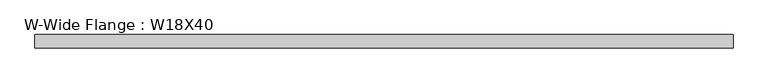
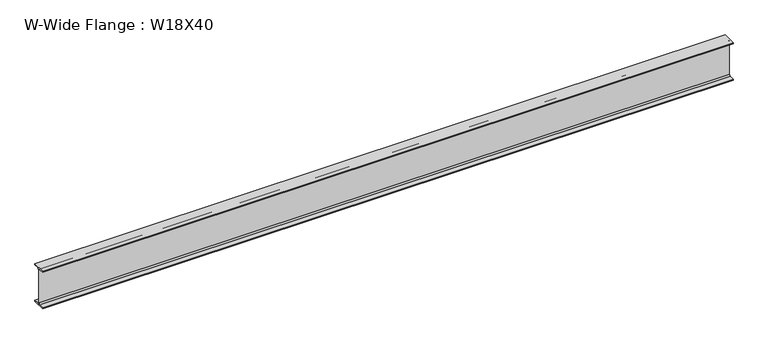
"""IFC4 building model written with IfcOpenShell, lengths in millimetres: beam geometry, W-Wide Flange : W18X40."""

from ifc_helpers import new_model, si_unit, point, frame, frame_2d, origin, place, context, project, spatial, polyline, circle_curve, trimmed, segment, composite_curve, outline, extrude, source, transform, mapped, element, save


def w_wide_flange_w18x40_d8d7ebc0(model_context):
    return source(origin(), model_context, "Body", "SweptSolid", [
        extrude(outline(composite_curve([segment(polyline([(76.454, -213.995), (76.454, -227.33), (-76.454, -227.33), (-76.454, -213.995), (-20.828, -213.995)]), True, "CONTINUOUS"), segment(trimmed(circle_curve(frame_2d((-20.828, -197.1675)), 16.8275), [point((-20.828, -213.995))], [point((-4.0005, -197.1675))], True, "CARTESIAN"), True, "CONTINUOUS"), segment(polyline([(-4.0005, -197.1675), (-4.0005, 197.1675)]), True, "CONTINUOUS"), segment(trimmed(circle_curve(frame_2d((-20.828, 197.1675)), 16.8275), [point((-4.0005, 197.1675))], [point((-20.828, 213.995))], True, "CARTESIAN"), True, "CONTINUOUS"), segment(polyline([(-20.828, 213.995), (-76.454, 213.995), (-76.454, 227.33), (76.454, 227.33), (76.454, 213.995), (20.828, 213.995)]), True, "CONTINUOUS"), segment(trimmed(circle_curve(frame_2d((20.828, 197.1675)), 16.8275), [point((20.828, 213.995))], [point((4.0005, 197.1675))], True, "CARTESIAN"), True, "CONTINUOUS"), segment(polyline([(4.0005, 197.1675), (4.0005, -197.1675)]), True, "CONTINUOUS"), segment(trimmed(circle_curve(frame_2d((20.828, -197.1675)), 16.8275), [point((4.0005, -197.1675))], [point((20.828, -213.995))], True, "CARTESIAN"), True, "CONTINUOUS"), segment(polyline([(20.828, -213.995), (76.454, -213.995)]), True, "CONTINUOUS")], self_intersect=False)), frame((-3923.03, 0.0, 0.0), z_axis=(1.0, 0.0, 0.0), x_axis=(0.0, 1.0, 0.0)), (0.0, 0.0, 1.0), 7902.8925),
    ])


if __name__ == "__main__":
    model = new_model("IFC4")
    model_context = context("Model", 3, world=origin())
    ifc_project = project(units=[si_unit("LENGTHUNIT", "METRE", prefix="MILLI")], contexts=[model_context])
    site = spatial("IfcSite", under=ifc_project)
    building = spatial("IfcBuilding", under=site)
    placement = place(None, origin())
    w_wide_flange_w18x40_shape = w_wide_flange_w18x40_d8d7ebc0(model_context)
    element("IfcBeam", 1, ObjectType="W-Wide Flange : W18X40", at=placement, inside=building, context=model_context, shape_type="MappedRepresentation", body=[
        mapped(w_wide_flange_w18x40_shape, transform((0.0, 0.0, 0.0), x_axis=(1.0, 0.0, 0.0), y_axis=(0.0, 1.0, 0.0), z_axis=(0.0, 0.0, 1.0))),
    ])
    save(model, "model.ifc")

# Revit data of these elements
# Type "W-Wide Flange : W18X40"
#   Assembly Code = "B10"
#   W = 40
#   Length [instance default] = 5' - 0"
#   bf = 0' - 6.02"
#   d = 1' - 5.9"
#   k = 0' - 1 3/16"
#   k2 = 0' - 0.6625"
#   tf = 0' - 0.525"
#   tw = 0' - 0.315"
#   A = 0.0819444 SF
#   Structural Material [instance default] = Steel ASTM A992
# Element 1 (IfcBeam, "W-Wide Flange : W18X40")
#   Materials on its faces: "Steel ASTM A992"
# Materials
#   "Steel ASTM A992": class "Metal", colour RGB 199 199 199, transparency 0, Description = "Structural steel 50ksi", Cost = 0
